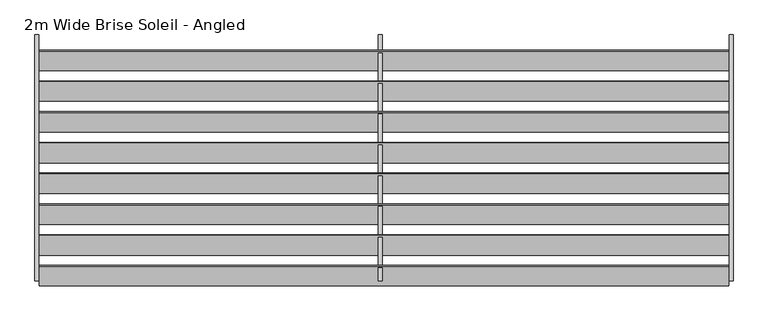
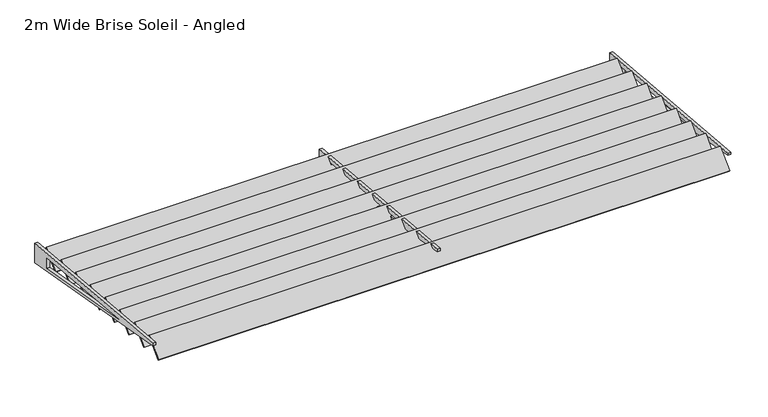
"""IFC4 building model written with IfcOpenShell, lengths in millimetres: railing geometry, 2m Wide Brise Soleil - Angled."""

from ifc_helpers import new_model, si_unit, frame, origin, place, context, project, spatial, polyline, outline, extrude, source, transform, mapped, element, save


def railing_2m_wide_brise_soleil_angled_944c0c30(model_context):
    return source(origin(), model_context, "Body", "SweptSolid", [
        extrude(outline(polyline([(0.0, -10.0000001), (0.0, 0.0), (5596.1382149, 0.0), (5596.1382149, -10.0000001), (0.0, -10.0000001)])), frame((4432.3404491, -35753.4041502, 10.034106), z_axis=(0.0, 0.7071067811931987, 0.7071067811798963), x_axis=(1.0, 0.0, 0.0)), (0.0, 0.0, 1.0), 225.0),
        extrude(outline(polyline([(0.0, -10.0000001), (0.0, 0.0), (5596.1382149, 0.0), (5596.1382149, -10.0000001), (0.0, -10.0000001)])), frame((4432.3404491, -35503.4041502, -9.965894), z_axis=(0.0, 0.7071067811931987, 0.7071067811798963), x_axis=(1.0, 0.0, 0.0)), (0.0, 0.0, 1.0), 225.0),
        extrude(outline(polyline([(0.0, -10.0000001), (0.0, 0.0), (5596.1382149, 0.0), (5596.1382149, -10.0000001), (0.0, -10.0000001)])), frame((4432.3404491, -35253.4041502, -31.965894), z_axis=(0.0, 0.7071067811931987, 0.7071067811798963), x_axis=(1.0, 0.0, 0.0)), (0.0, 0.0, 1.0), 225.0),
        extrude(outline(polyline([(0.0, -10.0000001), (0.0, 0.0), (5596.1382149, 0.0), (5596.1382149, -10.0000001), (0.0, -10.0000001)])), frame((4432.3404491, -35003.4041502, -53.965894), z_axis=(0.0, 0.7071067811931987, 0.7071067811798963), x_axis=(1.0, 0.0, 0.0)), (0.0, 0.0, 1.0), 225.0),
        extrude(outline(polyline([(0.0, -10.0000001), (0.0, 0.0), (5596.1382149, 0.0), (5596.1382149, -10.0000001), (0.0, -10.0000001)])), frame((4432.3404491, -34753.4041502, -75.965894), z_axis=(0.0, 0.7071067811931987, 0.7071067811798963), x_axis=(1.0, 0.0, 0.0)), (0.0, 0.0, 1.0), 225.0),
        extrude(outline(polyline([(0.0, -10.0000001), (0.0, 0.0), (5596.1382149, 0.0), (5596.1382149, -10.0000001), (0.0, -10.0000001)])), frame((4432.3404491, -34503.4041502, -97.965894), z_axis=(0.0, 0.7071067811931987, 0.7071067811798963), x_axis=(1.0, 0.0, 0.0)), (0.0, 0.0, 1.0), 225.0),
        extrude(outline(polyline([(0.0, -10.0000001), (0.0, 0.0), (5596.1382149, 0.0), (5596.1382149, -10.0000001), (0.0, -10.0000001)])), frame((4432.3404491, -34253.4041502, -118.965894), z_axis=(0.0, 0.7071067811931987, 0.7071067811798963), x_axis=(1.0, 0.0, 0.0)), (0.0, 0.0, 1.0), 225.0),
        extrude(outline(polyline([(0.0, -10.0000001), (0.0, 0.0), (5596.1382149, 0.0), (5596.1382149, -10.0000001), (0.0, -10.0000001)])), frame((4432.3404491, -34003.4041502, -139.965894), z_axis=(0.0, 0.7071067811931987, 0.7071067811798963), x_axis=(1.0, 0.0, 0.0)), (0.0, 0.0, 1.0), 225.0),
        extrude(outline(polyline([(-35720.1943586, 174.9773271), (-33720.1943586, 0.0), (-33720.1943586, -200.0), (-35720.1943586, 149.9773271), (-35720.1943586, 174.9773271)]), holes=[polyline([(-33920.1943586, -139.6223905), (-33920.1943586, -32.6932592), (-35142.2415739, 74.2220185), (-33920.1943586, -139.6223905)])]), frame((7184.5476938, 0.0, 0.0), z_axis=(1.0, 0.0, 0.0), x_axis=(0.0, 1.0, 0.0)), (0.0, 0.0, 1.0), 30.0),
        extrude(outline(polyline([(-35720.1943586, 174.9773271), (-33720.1943586, 0.0), (-33720.1943586, -200.0), (-35720.1943586, 149.9773271), (-35720.1943586, 174.9773271)]), holes=[polyline([(-33920.1943586, -139.6223905), (-33920.1943586, -32.6932592), (-35142.2415739, 74.2220185), (-33920.1943586, -139.6223905)])]), frame((10032.6168013, 0.0, 0.0), z_axis=(1.0, 0.0, 0.0), x_axis=(0.0, 1.0, 0.0)), (0.0, 0.0, 1.0), 30.0),
        extrude(outline(polyline([(-35720.1943586, 174.9773271), (-33720.1943586, 0.0), (-33720.1943586, -200.0), (-35720.1943586, 149.9773271), (-35720.1943586, 174.9773271)]), holes=[polyline([(-33920.1943586, -139.6223905), (-33920.1943586, -32.6932592), (-35142.2415739, 74.2220185), (-33920.1943586, -139.6223905)])]), frame((4396.4785864, 0.0, 0.0), z_axis=(1.0, 0.0, 0.0), x_axis=(0.0, 1.0, 0.0)), (0.0, 0.0, 1.0), 30.0),
    ])


if __name__ == "__main__":
    model = new_model("IFC4")
    model_context = context("Model", 3, world=origin())
    ifc_project = project(units=[si_unit("LENGTHUNIT", "METRE", prefix="MILLI")], contexts=[model_context])
    site = spatial("IfcSite", under=ifc_project)
    building = spatial("IfcBuilding", under=site)
    placement = place(None, origin())
    railing_2m_wide_brise_soleil_angled_shape = railing_2m_wide_brise_soleil_angled_944c0c30(model_context)
    element("IfcRailing", 1, ObjectType="2m Wide Brise Soleil - Angled", at=placement, inside=building, context=model_context, shape_type="MappedRepresentation", body=[
        mapped(railing_2m_wide_brise_soleil_angled_shape, transform((0.0, 0.0, 0.0), x_axis=(1.0, 0.0, 0.0), y_axis=(0.0, 1.0, 0.0), z_axis=(0.0, 0.0, 1.0))),
    ])
    save(model, "model.ifc")

# Revit data of these elements
# Element 1 (IfcRailing, "2m Wide Brise Soleil - Angled")
#   Materials on its faces: "Metal - Aluminium", "Metal - Steel"
# Materials
#   "Metal - Aluminium": class "Unassigned", colour RGB 247 247 247, transparency 0
#   "Metal - Steel": class "Unassigned", colour RGB 199 199 199, transparency 0
